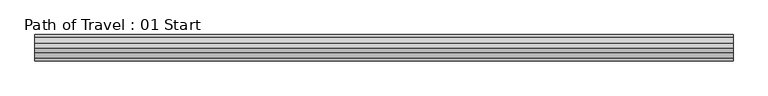
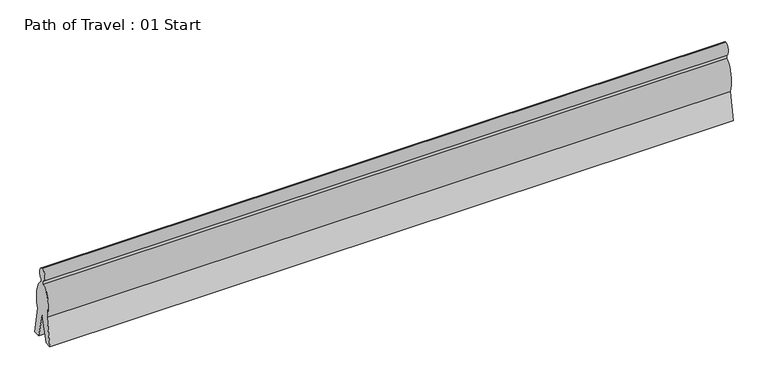
"""IFC4 building model written with IfcOpenShell, lengths in millimetres: proxy geometry, Path of Travel : 01 Start."""

from ifc_helpers import new_model, si_unit, point, frame, origin, place, context, project, spatial, ellipse_curve, trimmed, source, transform, mapped, element, save
from ifc_brep_helpers import plane_surface, extruded_surface, advanced_brep


def path_of_travel_01_start_b18a8849(model_context):
    return source(origin(), model_context, "Body", "AdvancedBrep", [
        advanced_brep(
        [(227.5554837, 0.0, 1727.2), (227.5554837, 42.9018657, 1436.6534209), (227.5554837, 42.9018657, 1363.4763406), (227.5554837, 184.1186263, 643.4144547), (227.5554837, 297.5699544, 0.0), (227.5554837, 145.6574193, 0.0), (227.5554837, 0.0, 584.2), (227.5554837, -145.6574193, 0.0), (227.5554837, -297.5699544, 0.0), (227.5554837, -184.1186263, 643.4144547), (227.5554837, -42.9018657, 1363.4763406), (227.5554837, -42.9018657, 1436.6534209), (15924.7554837, 0.0, 1727.2), (15924.7554837, -42.9018657, 1436.6534209), (15924.7554837, -42.9018657, 1363.4763406), (15924.7554837, -184.1186263, 643.4144547), (15924.7554837, -297.5699544, 0.0), (15924.7554837, -145.6574193, 0.0), (15924.7554837, 0.0, 584.2), (15924.7554837, 145.6574193, 0.0), (15924.7554837, 297.5699544, 0.0), (15924.7554837, 184.1186263, 643.4144547), (15924.7554837, 42.9018657, 1363.4763406), (15924.7554837, 42.9018657, 1436.6534209)],
        [
            (0, 1, ellipse_curve(frame((227.5554837, 0.0, 1574.8), z_axis=(-1.0, 0.0, 0.0), x_axis=(0.0, 0.0, 1.0)), 152.4, 101.6)),
            (1, 2),
            (2, 3, ellipse_curve(frame((227.5554837, 0.0, 914.4), z_axis=(-1.0, 0.0, 0.0), x_axis=(0.0, 0.0, -1.0)), 457.2, 228.6)),
            (3, 4),
            (4, 5),
            (5, 6),
            (6, 7),
            (7, 8),
            (8, 9),
            (9, 10, ellipse_curve(frame((227.5554837, 0.0, 914.4), z_axis=(-1.0, 0.0, 0.0), x_axis=(0.0, 0.0, -1.0)), 457.2, 228.6)),
            (10, 11),
            (11, 0, ellipse_curve(frame((227.5554837, 0.0, 1574.8), z_axis=(-1.0, 0.0, 0.0), x_axis=(0.0, 0.0, 1.0)), 152.4, 101.6)),
            (12, 13, ellipse_curve(frame((15924.7554837, 0.0, 1574.8), z_axis=(1.0, 0.0, 0.0), x_axis=(0.0, 0.0, 1.0)), 152.4, 101.6)),
            (13, 14),
            (14, 15, ellipse_curve(frame((15924.7554837, 0.0, 914.4), z_axis=(1.0, 0.0, 0.0), x_axis=(0.0, 0.0, -1.0)), 457.2, 228.6)),
            (15, 16),
            (16, 17),
            (17, 18),
            (18, 19),
            (19, 20),
            (20, 21),
            (21, 22, ellipse_curve(frame((15924.7554837, 0.0, 914.4), z_axis=(1.0, 0.0, 0.0), x_axis=(0.0, 0.0, -1.0)), 457.2, 228.6)),
            (22, 23),
            (23, 12, ellipse_curve(frame((15924.7554837, 0.0, 1574.8), z_axis=(1.0, 0.0, 0.0), x_axis=(0.0, 0.0, 1.0)), 152.4, 101.6)),
            (0, 12),
            (23, 1),
            (22, 2),
            (21, 3),
            (20, 4),
            (19, 5),
            (18, 6),
            (17, 7),
            (16, 8),
            (15, 9),
            (14, 10),
            (13, 11),
        ],
        [
            plane_surface(frame((227.5554837, 0.0, 0.0), z_axis=(-1.0, 0.0, 0.0), x_axis=(0.0, 0.0, 1.0))),
            plane_surface(frame((15924.7554837, 0.0, 0.0), z_axis=(1.0, 0.0, 0.0), x_axis=(0.0, 0.0, 1.0))),
            extruded_surface(trimmed(ellipse_curve(frame((15924.7554837, 0.0, 1574.8), z_axis=(-1.0, 0.0, 0.0), x_axis=(0.0, 0.0, 1.0)), 152.4, 101.6), [point((15924.7554837, 0.0, 1727.2))], [point((15924.7554837, 42.9018657, 1436.6534209))], True, "CARTESIAN"), (-15697.2, 0.0, 0.0), 15697.2),
            plane_surface(frame((227.5554837, 42.9018657, 1436.6534209), z_axis=(0.0, 1.0, 0.0), x_axis=(1.0, 0.0, 0.0))),
            extruded_surface(trimmed(ellipse_curve(frame((15924.7554837, 0.0, 914.4), z_axis=(-1.0, 0.0, 0.0), x_axis=(0.0, 0.0, -1.0)), 457.2, 228.6), [point((15924.7554837, 42.9018657, 1363.4763406))], [point((15924.7554837, 184.1186263, 643.4144547))], True, "CARTESIAN"), (-15697.2, 0.0, 0.0), 15697.2),
            plane_surface(frame((227.5554837, 184.1186263, 643.4144547), z_axis=(0.0, 0.9848077530122078, 0.17364817766693205), x_axis=(1.0, 0.0, 0.0))),
            plane_surface(frame((227.5554837, 297.5699544, 0.0), z_axis=(0.0, 0.0, -1.0), x_axis=(1.0, 0.0, 0.0))),
            plane_surface(frame((227.5554837, 145.6574193, 0.0), z_axis=(0.0, -0.9702957262760199, -0.2419218955995739), x_axis=(1.0, 0.0, 0.0))),
            plane_surface(frame((227.5554837, 0.0, 584.2), z_axis=(0.0, 0.9702957262759961, -0.24192189559966923), x_axis=(1.0, 0.0, 0.0))),
            plane_surface(frame((227.5554837, -145.6574193, 0.0), z_axis=(0.0, 0.0, -1.0), x_axis=(1.0, 0.0, 0.0))),
            plane_surface(frame((227.5554837, -297.5699544, 0.0), z_axis=(0.0, -0.984807753012208, 0.17364817766693066), x_axis=(1.0, 0.0, 0.0))),
            extruded_surface(trimmed(ellipse_curve(frame((15924.7554837, 0.0, 914.4), z_axis=(-1.0, 0.0, 0.0), x_axis=(0.0, 0.0, -1.0)), 457.2, 228.6), [point((15924.7554837, -184.1186263, 643.4144547))], [point((15924.7554837, -42.9018657, 1363.4763406))], True, "CARTESIAN"), (-15697.2, 0.0, 0.0), 15697.2),
            plane_surface(frame((227.5554837, -42.9018657, 1363.4763406), z_axis=(0.0, -1.0, 0.0), x_axis=(1.0, 0.0, 0.0))),
            extruded_surface(trimmed(ellipse_curve(frame((15924.7554837, 0.0, 1574.8), z_axis=(-1.0, 0.0, 0.0), x_axis=(0.0, 0.0, 1.0)), 152.4, 101.6), [point((15924.7554837, -42.9018657, 1436.6534209))], [point((15924.7554837, 0.0, 1727.2))], True, "CARTESIAN"), (-15697.2, 0.0, 0.0), 15697.2),
        ],
        [
            (0, [[1, 2, 3, 4, 5, 6, 7, 8, 9, 10, 11, 12]]),
            (1, [[13, 14, 15, 16, 17, 18, 19, 20, 21, 22, 23, 24]]),
            (2, [[-1, 25, -24, 26]]),
            (3, [[-2, -26, -23, 27]]),
            (4, [[-3, -27, -22, 28]]),
            (5, [[-4, -28, -21, 29]]),
            (6, [[-5, -29, -20, 30]]),
            (7, [[-6, -30, -19, 31]]),
            (8, [[-7, -31, -18, 32]]),
            (9, [[-8, -32, -17, 33]]),
            (10, [[-9, -33, -16, 34]]),
            (11, [[-10, -34, -15, 35]]),
            (12, [[-11, -35, -14, 36]]),
            (13, [[-12, -36, -13, -25]]),
        ],
    ),
    ])


if __name__ == "__main__":
    model = new_model("IFC4")
    model_context = context("Model", 3, world=origin())
    ifc_project = project(units=[si_unit("LENGTHUNIT", "METRE", prefix="MILLI")], contexts=[model_context])
    site = spatial("IfcSite", under=ifc_project)
    building = spatial("IfcBuilding", under=site)
    placement = place(None, origin())
    path_of_travel_01_start_shape = path_of_travel_01_start_b18a8849(model_context)
    element("IfcBuildingElementProxy", 1, Name="Path of Travel : 01 Start", ObjectType="Path of Travel : 01 Start", at=placement, inside=building, context=model_context, shape_type="MappedRepresentation", body=[
        mapped(path_of_travel_01_start_shape, transform((0.0, 0.0, 0.0), x_axis=(1.0, 0.0, 0.0), y_axis=(0.0, 1.0, 0.0), z_axis=(0.0, 0.0, 1.0))),
    ])
    save(model, "model.ifc")

# Revit data of these elements
# Type "Path of Travel : 01 Start"
#   Path of Egress [instance default] = 4' - 0"
#   built-in parameter 1001306 [instance default] = 4 (stored number, unit not read)
#   Dot at Start = yes
#   Arrow in Middle = yes
#   Arrow at End = no
#   Egress Path = none
# Element 1 (IfcBuildingElementProxy, "Path of Travel : 01 Start")
#   Path of Egress = 51' - 6"
#   built-in parameter 1001306 = 51.5 (stored number, unit not read)
#   Materials on its faces: "Egress Path Solid"
# Materials
#   "Egress Path Solid": class "Unassigned", colour RGB 255 128 64, transparency 0.75, Comments = "Rendering appearance not upgraded "
